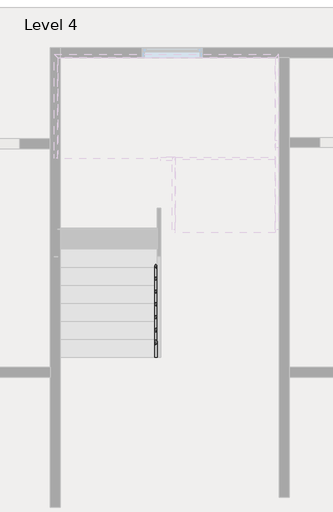
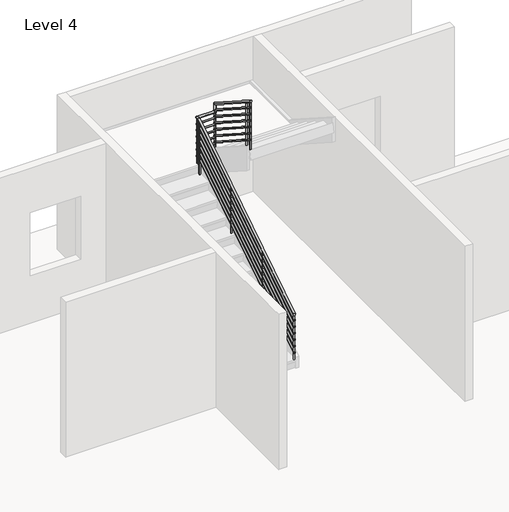
# One storey, part 6 of 7: 1 railing.
"""IFC4 building model written with IfcOpenShell, lengths in millimetres."""

from ifc_helpers import new_model, si_unit, point, frame, frame_2d, origin, place, context, project, spatial, circle_curve, ellipse_curve, trimmed, segment, composite_curve, outline, extrude, element, save
from ifc_brep_helpers import plane_surface, cylinder_surface, advanced_brep

model = new_model("IFC4")

# Units and contexts
model_context = context("Model", 3, world=origin())
ifc_project = project(units=[si_unit("LENGTHUNIT", "METRE", prefix="MILLI")], contexts=[model_context])

# Site, building, storey
site = spatial("IfcSite", under=ifc_project)
building = spatial("IfcBuilding", under=site)
storey = spatial("IfcBuildingStorey", under=building, Name="Level 4", Elevation=9500.0)

# Railing
placement = place(None, origin())
element("IfcRailing", 1, ObjectType="900mm Pipe", at=placement, inside=storey, context=model_context, shape_type="SolidModel", body=[
    advanced_brep(
    [(-504.8393676, 4284.7509075, 10552.7068065), (-544.8393676, 4284.7509075, 10552.7068065), (-504.8393676, 7315.616134, 12497.6470588), (-544.8393676, 7315.616134, 12497.6470588), (-504.8393676, 7337.8781803, 12497.6470588), (-544.8393676, 7377.8781803, 12497.6470588), (-201.3120949, 7337.8781803, 12497.6470588), (-201.3120949, 7377.8781803, 12497.6470588)],
    [
        (0, 1, ellipse_curve(frame((-524.8393676, 4284.7509075, 10552.7068065), z_axis=(0.0, -1.0, 0.0), x_axis=(0.0, 0.0, -1.0)), 23.7637817, 20.0)),
        (1, 0, ellipse_curve(frame((-524.8393676, 4284.7509075, 10552.7068065), z_axis=(0.0, -1.0, 0.0), x_axis=(0.0, 0.0, -1.0)), 23.7637817, 20.0)),
        (0, 2),
        (2, 3, ellipse_curve(frame((-524.8393676, 7315.616134, 12497.6470588), z_axis=(0.0, -0.9595876426002529, -0.28140994326585084), x_axis=(0.0, 0.2814099432658509, -0.959587642600253)), 20.8422859, 20.0)),
        (3, 1),
        (3, 2, ellipse_curve(frame((-524.8393676, 7315.616134, 12497.6470588), z_axis=(0.0, -0.9595876426002529, -0.28140994326585084), x_axis=(0.0, 0.2814099432658509, -0.959587642600253)), 20.8422859, 20.0)),
        (2, 4),
        (4, 5, ellipse_curve(frame((-524.8393676, 7357.8781803, 12497.6470588), z_axis=(-0.7071067811865475, -0.7071067811865475, 0.0), x_axis=(0.7071067811865474, -0.7071067811865476, 0.0)), 28.2842712, 20.0)),
        (5, 3),
        (5, 4, ellipse_curve(frame((-524.8393676, 7357.8781803, 12497.6470588), z_axis=(-0.7071067811865475, -0.7071067811865475, 0.0), x_axis=(0.7071067811865474, -0.7071067811865476, 0.0)), 28.2842712, 20.0)),
        (6, 7, ellipse_curve(frame((-201.3120949, 7357.8781803, 12497.6470588), z_axis=(0.7071067811865476, 0.0, 0.7071067811865476), x_axis=(-0.7071067811865474, 0.0, 0.7071067811865476)), 28.2842712, 20.0)),
        (7, 6, ellipse_curve(frame((-201.3120949, 7357.8781803, 12497.6470588), z_axis=(0.7071067811865476, 0.0, 0.7071067811865476), x_axis=(-0.7071067811865474, 0.0, 0.7071067811865476)), 28.2842712, 20.0)),
        (4, 6),
        (7, 5),
    ],
    [
        plane_surface(frame((-524.8393676, 4284.7509075, 10576.4705882), z_axis=(0.0, -1.0, 0.0), x_axis=(0.0, 0.0, 1.0))),
        cylinder_surface(frame((-524.8393676, 4295.5524077, 10559.6382505), z_axis=(0.0, -0.8416168876622212, -0.5400750081254975), x_axis=(-1.0, 0.0, 0.0)), 20.0),
        cylinder_surface(frame((-524.8393676, 7309.7509075, 12497.6470588), z_axis=(0.0, -1.0, 0.0), x_axis=(-1.0, 0.0, 0.0)), 20.0),
        plane_surface(frame((-221.3120949, 7357.8781803, 12517.6470588), z_axis=(0.7071067811865476, 0.0, 0.7071067811865476), x_axis=(0.7071067811865476, 0.0, -0.7071067811865476))),
        cylinder_surface(frame((-524.8393676, 7357.8781803, 12497.6470588), z_axis=(-1.0, 0.0, 0.0), x_axis=(0.0, 1.0, 0.0)), 20.0),
    ],
    [
        (0, [[1, 2]]),
        (1, [[-1, 3, 4, 5]]),
        (1, [[-2, -5, 6, -3]]),
        (2, [[-4, 7, 8, 9]]),
        (2, [[-6, -9, 10, -7]]),
        (3, [[11, 12]]),
        (4, [[-8, 13, -12, 14]]),
        (4, [[-10, -14, -11, -13]]),
    ],
),
    advanced_brep(
    [(-201.3120949, 7337.8781803, 12497.6470588), (-201.3120949, 7377.8781803, 12497.6470588), (-201.3120949, 7337.8781803, 12643.124843), (-201.3120949, 7377.8781803, 12664.9839572)],
    [
        (0, 1, ellipse_curve(frame((-201.3120949, 7357.8781803, 12497.6470588), z_axis=(-0.7071067811865476, 0.0, -0.7071067811865476), x_axis=(0.7071067811865476, 0.0, -0.7071067811865474)), 28.2842712, 20.0)),
        (1, 0, ellipse_curve(frame((-201.3120949, 7357.8781803, 12497.6470588), z_axis=(-0.7071067811865476, 0.0, -0.7071067811865476), x_axis=(0.7071067811865476, 0.0, -0.7071067811865474)), 28.2842712, 20.0)),
        (2, 3, ellipse_curve(frame((-201.3120949, 7357.8781803, 12654.0544001), z_axis=(0.0, -0.47954405004884676, 0.877517808402057), x_axis=(0.0, -0.8775178084020571, -0.47954405004884676)), 22.7915602, 20.0)),
        (3, 2, ellipse_curve(frame((-201.3120949, 7357.8781803, 12654.0544001), z_axis=(0.0, -0.47954405004884676, 0.877517808402057), x_axis=(0.0, -0.8775178084020571, -0.47954405004884676)), 22.7915602, 20.0)),
        (0, 2),
        (3, 1),
    ],
    [
        plane_surface(frame((-201.3120949, 7357.8781803, 12497.6470588), z_axis=(-0.7071067811865476, 0.0, -0.7071067811865476), x_axis=(0.7071067811865476, 0.0, -0.7071067811865476))),
        plane_surface(frame((-201.3120949, 7357.8781803, 12654.0544001), z_axis=(0.0, -0.47954405004884676, 0.877517808402057), x_axis=(1.0, 0.0, 0.0))),
        cylinder_surface(frame((-201.3120949, 7357.8781803, 12497.6470588), z_axis=(0.0, 0.0, -1.0), x_axis=(0.0, 1.0, 0.0)), 20.0),
    ],
    [
        (0, [[1, 2]]),
        (1, [[3, 4]]),
        (2, [[-1, 5, -4, 6]]),
        (2, [[-2, -6, -3, -5]]),
    ],
),
    advanced_brep(
    [(-221.3120949, 7357.8781803, 12654.0544001), (-181.3120949, 7357.8781803, 12654.0544001), (-221.3120949, 6232.4781803, 13376.2362183), (-181.3120949, 6232.4781803, 13376.2362183)],
    [
        (0, 1, ellipse_curve(frame((-201.3120949, 7357.8781803, 12654.0544001), z_axis=(0.0, 0.47954405004884676, -0.877517808402057), x_axis=(0.0, 0.8775178084020568, 0.47954405004884676)), 22.7915602, 20.0)),
        (1, 0, ellipse_curve(frame((-201.3120949, 7357.8781803, 12654.0544001), z_axis=(0.0, 0.47954405004884676, -0.877517808402057), x_axis=(0.0, 0.8775178084020568, 0.47954405004884676)), 22.7915602, 20.0)),
        (2, 3, ellipse_curve(frame((-201.3120949, 6232.4781803, 13376.2362183), z_axis=(0.0, -1.0, 0.0), x_axis=(0.0, 0.0, -1.0)), 23.7637817, 20.0)),
        (3, 2, ellipse_curve(frame((-201.3120949, 6232.4781803, 13376.2362183), z_axis=(0.0, -1.0, 0.0), x_axis=(0.0, 0.0, -1.0)), 23.7637817, 20.0)),
        (0, 2),
        (3, 1),
    ],
    [
        plane_surface(frame((-201.3120949, 7377.8781803, 12664.9839572), z_axis=(0.0, 0.47954405004884676, -0.877517808402057), x_axis=(1.0, 0.0, 0.0))),
        plane_surface(frame((-201.3120949, 6232.4781803, 13400.0), z_axis=(0.0, -1.0, 0.0), x_axis=(0.0, 0.0, -1.0))),
        cylinder_surface(frame((-201.3120949, 7367.0766801, 12648.1516195), z_axis=(0.0, 0.8416168876622208, -0.5400750081254984), x_axis=(1.0, 0.0, 0.0)), 20.0),
    ],
    [
        (0, [[1, 2]]),
        (1, [[3, 4]]),
        (2, [[-1, 5, -4, 6]]),
        (2, [[-2, -6, -3, -5]]),
    ],
),
    advanced_brep(
    [(-539.8393676, 4284.7509075, 10433.647752), (-509.8393676, 4284.7509075, 10433.647752), (-539.8393676, 7309.7509075, 12374.8242225), (-509.8393676, 7309.7509075, 12374.8242225)],
    [
        (0, 1, ellipse_curve(frame((-524.8393676, 4284.7509075, 10433.647752), z_axis=(0.0, -1.0, 0.0), x_axis=(0.0, 0.0, -1.0)), 17.8228363, 15.0)),
        (1, 0, ellipse_curve(frame((-524.8393676, 4284.7509075, 10433.647752), z_axis=(0.0, -1.0, 0.0), x_axis=(0.0, 0.0, -1.0)), 17.8228363, 15.0)),
        (2, 3, ellipse_curve(frame((-524.8393676, 7309.7509075, 12374.8242225), z_axis=(0.0, 1.0, 0.0), x_axis=(0.0, 0.0, -1.0)), 17.8228363, 15.0)),
        (3, 2, ellipse_curve(frame((-524.8393676, 7309.7509075, 12374.8242225), z_axis=(0.0, 1.0, 0.0), x_axis=(0.0, 0.0, -1.0)), 17.8228363, 15.0)),
        (0, 2),
        (3, 1),
    ],
    [
        plane_surface(frame((-524.8393676, 4284.7509075, 10451.4705882), z_axis=(0.0, -1.0, 0.0), x_axis=(0.0, 0.0, 1.0))),
        plane_surface(frame((-524.8393676, 7309.7509075, 12392.6470588), z_axis=(0.0, 1.0, 0.0), x_axis=(0.0, 0.0, 1.0))),
        cylinder_surface(frame((-524.8393676, 4292.8520327, 10438.8463349), z_axis=(0.0, -0.8416168876622212, -0.5400750081254975), x_axis=(1.0, 0.0, 0.0)), 15.0),
    ],
    [
        (0, [[1, 2]]),
        (1, [[3, 4]]),
        (2, [[-1, 5, -4, 6]]),
        (2, [[-2, -6, -3, -5]]),
    ],
),
    advanced_brep(
    [(-539.8393676, 7309.7509075, 12377.6470588), (-509.8393676, 7309.7509075, 12377.6470588), (-539.8393676, 7342.8781803, 12377.6470588), (-509.8393676, 7342.8781803, 12377.6470588)],
    [
        (0, 1, circle_curve(frame((-524.8393676, 7309.7509075, 12377.6470588), z_axis=(0.0, -1.0, 0.0), x_axis=(1.0, 0.0, 0.0)), 15.0)),
        (1, 0, circle_curve(frame((-524.8393676, 7309.7509075, 12377.6470588), z_axis=(0.0, -1.0, 0.0), x_axis=(1.0, 0.0, 0.0)), 15.0)),
        (2, 3, circle_curve(frame((-524.8393676, 7342.8781803, 12377.6470588), z_axis=(0.0, 1.0, 0.0), x_axis=(1.0, 0.0, 0.0)), 15.0)),
        (3, 2, circle_curve(frame((-524.8393676, 7342.8781803, 12377.6470588), z_axis=(0.0, 1.0, 0.0), x_axis=(1.0, 0.0, 0.0)), 15.0)),
        (0, 2),
        (3, 1),
    ],
    [
        plane_surface(frame((-524.8393676, 7309.7509075, 12392.6470588), z_axis=(0.0, -1.0, 0.0), x_axis=(0.0, 0.0, 1.0))),
        plane_surface(frame((-524.8393676, 7342.8781803, 12392.6470588), z_axis=(0.0, 1.0, 0.0), x_axis=(0.0, 0.0, 1.0))),
        cylinder_surface(frame((-524.8393676, 7309.7509075, 12377.6470588), z_axis=(0.0, -1.0, 0.0), x_axis=(1.0, 0.0, 0.0)), 15.0),
    ],
    [
        (0, [[1, 2]]),
        (1, [[3, 4]]),
        (2, [[-1, 5, -4, 6]]),
        (2, [[-2, -6, -3, -5]]),
    ],
),
    advanced_brep(
    [(-539.8393676, 7372.8781803, 12377.6470588), (-539.8393676, 7342.8781803, 12377.6470588), (-216.3120949, 7372.8781803, 12377.6470588), (-216.3120949, 7342.8781803, 12377.6470588)],
    [
        (0, 1, circle_curve(frame((-539.8393676, 7357.8781803, 12377.6470588), z_axis=(-1.0, 0.0, 0.0), x_axis=(0.0, -1.0, 0.0)), 15.0)),
        (1, 0, circle_curve(frame((-539.8393676, 7357.8781803, 12377.6470588), z_axis=(-1.0, 0.0, 0.0), x_axis=(0.0, -1.0, 0.0)), 15.0)),
        (2, 3, circle_curve(frame((-216.3120949, 7357.8781803, 12377.6470588), z_axis=(1.0, 0.0, 0.0), x_axis=(0.0, -1.0, 0.0)), 15.0)),
        (3, 2, circle_curve(frame((-216.3120949, 7357.8781803, 12377.6470588), z_axis=(1.0, 0.0, 0.0), x_axis=(0.0, -1.0, 0.0)), 15.0)),
        (0, 2),
        (3, 1),
    ],
    [
        plane_surface(frame((-539.8393676, 7357.8781803, 12392.6470588), z_axis=(-1.0, 0.0, 0.0), x_axis=(0.0, 1.0, 0.0))),
        plane_surface(frame((-216.3120949, 7357.8781803, 12392.6470588), z_axis=(1.0, 0.0, 0.0), x_axis=(0.0, 1.0, 0.0))),
        cylinder_surface(frame((-539.8393676, 7357.8781803, 12377.6470588), z_axis=(-1.0, 0.0, 0.0), x_axis=(0.0, -1.0, 0.0)), 15.0),
    ],
    [
        (0, [[1, 2]]),
        (1, [[3, 4]]),
        (2, [[-1, 5, -4, 6]]),
        (2, [[-2, -6, -3, -5]]),
    ],
),
    advanced_brep(
    [(-186.3120949, 7372.8781803, 12525.3696771), (-216.3120949, 7372.8781803, 12525.3696771), (-186.3120949, 6232.4781803, 13257.1771637), (-216.3120949, 6232.4781803, 13257.1771637)],
    [
        (0, 1, ellipse_curve(frame((-201.3120949, 7372.8781803, 12525.3696771), z_axis=(0.0, 1.0, 0.0), x_axis=(0.0, 0.0, -1.0)), 17.8228363, 15.0)),
        (1, 0, ellipse_curve(frame((-201.3120949, 7372.8781803, 12525.3696771), z_axis=(0.0, 1.0, 0.0), x_axis=(0.0, 0.0, -1.0)), 17.8228363, 15.0)),
        (2, 3, ellipse_curve(frame((-201.3120949, 6232.4781803, 13257.1771637), z_axis=(0.0, -1.0, 0.0), x_axis=(0.0, 0.0, -1.0)), 17.8228363, 15.0)),
        (3, 2, ellipse_curve(frame((-201.3120949, 6232.4781803, 13257.1771637), z_axis=(0.0, -1.0, 0.0), x_axis=(0.0, 0.0, -1.0)), 17.8228363, 15.0)),
        (0, 2),
        (3, 1),
    ],
    [
        plane_surface(frame((-201.3120949, 7372.8781803, 12543.1925134), z_axis=(0.0, 1.0, 0.0), x_axis=(0.0, 0.0, -1.0))),
        plane_surface(frame((-201.3120949, 6232.4781803, 13275.0), z_axis=(0.0, -1.0, 0.0), x_axis=(0.0, 0.0, -1.0))),
        cylinder_surface(frame((-201.3120949, 7364.7770552, 12530.5682601), z_axis=(0.0, 0.8416168876622208, -0.5400750081254984), x_axis=(-1.0, 0.0, 0.0)), 15.0),
    ],
    [
        (0, [[1, 2]]),
        (1, [[3, 4]]),
        (2, [[-1, 5, -4, 6]]),
        (2, [[-2, -6, -3, -5]]),
    ],
),
    advanced_brep(
    [(-539.8393676, 4284.7509075, 10308.647752), (-509.8393676, 4284.7509075, 10308.647752), (-539.8393676, 7309.7509075, 12249.8242225), (-509.8393676, 7309.7509075, 12249.8242225)],
    [
        (0, 1, ellipse_curve(frame((-524.8393676, 4284.7509075, 10308.647752), z_axis=(0.0, -1.0, 0.0), x_axis=(0.0, 0.0, -1.0)), 17.8228363, 15.0)),
        (1, 0, ellipse_curve(frame((-524.8393676, 4284.7509075, 10308.647752), z_axis=(0.0, -1.0, 0.0), x_axis=(0.0, 0.0, -1.0)), 17.8228363, 15.0)),
        (2, 3, ellipse_curve(frame((-524.8393676, 7309.7509075, 12249.8242225), z_axis=(0.0, 1.0, 0.0), x_axis=(0.0, 0.0, -1.0)), 17.8228363, 15.0)),
        (3, 2, ellipse_curve(frame((-524.8393676, 7309.7509075, 12249.8242225), z_axis=(0.0, 1.0, 0.0), x_axis=(0.0, 0.0, -1.0)), 17.8228363, 15.0)),
        (0, 2),
        (3, 1),
    ],
    [
        plane_surface(frame((-524.8393676, 4284.7509075, 10326.4705882), z_axis=(0.0, -1.0, 0.0), x_axis=(0.0, 0.0, 1.0))),
        plane_surface(frame((-524.8393676, 7309.7509075, 12267.6470588), z_axis=(0.0, 1.0, 0.0), x_axis=(0.0, 0.0, 1.0))),
        cylinder_surface(frame((-524.8393676, 4292.8520327, 10313.8463349), z_axis=(0.0, -0.8416168876622212, -0.5400750081254975), x_axis=(1.0, 0.0, 0.0)), 15.0),
    ],
    [
        (0, [[1, 2]]),
        (1, [[3, 4]]),
        (2, [[-1, 5, -4, 6]]),
        (2, [[-2, -6, -3, -5]]),
    ],
),
    advanced_brep(
    [(-539.8393676, 7309.7509075, 12252.6470588), (-509.8393676, 7309.7509075, 12252.6470588), (-539.8393676, 7342.8781803, 12252.6470588), (-509.8393676, 7342.8781803, 12252.6470588)],
    [
        (0, 1, circle_curve(frame((-524.8393676, 7309.7509075, 12252.6470588), z_axis=(0.0, -1.0, 0.0), x_axis=(1.0, 0.0, 0.0)), 15.0)),
        (1, 0, circle_curve(frame((-524.8393676, 7309.7509075, 12252.6470588), z_axis=(0.0, -1.0, 0.0), x_axis=(1.0, 0.0, 0.0)), 15.0)),
        (2, 3, circle_curve(frame((-524.8393676, 7342.8781803, 12252.6470588), z_axis=(0.0, 1.0, 0.0), x_axis=(1.0, 0.0, 0.0)), 15.0)),
        (3, 2, circle_curve(frame((-524.8393676, 7342.8781803, 12252.6470588), z_axis=(0.0, 1.0, 0.0), x_axis=(1.0, 0.0, 0.0)), 15.0)),
        (0, 2),
        (3, 1),
    ],
    [
        plane_surface(frame((-524.8393676, 7309.7509075, 12267.6470588), z_axis=(0.0, -1.0, 0.0), x_axis=(0.0, 0.0, 1.0))),
        plane_surface(frame((-524.8393676, 7342.8781803, 12267.6470588), z_axis=(0.0, 1.0, 0.0), x_axis=(0.0, 0.0, 1.0))),
        cylinder_surface(frame((-524.8393676, 7309.7509075, 12252.6470588), z_axis=(0.0, -1.0, 0.0), x_axis=(1.0, 0.0, 0.0)), 15.0),
    ],
    [
        (0, [[1, 2]]),
        (1, [[3, 4]]),
        (2, [[-1, 5, -4, 6]]),
        (2, [[-2, -6, -3, -5]]),
    ],
),
    advanced_brep(
    [(-539.8393676, 7372.8781803, 12252.6470588), (-539.8393676, 7342.8781803, 12252.6470588), (-216.3120949, 7372.8781803, 12252.6470588), (-216.3120949, 7342.8781803, 12252.6470588)],
    [
        (0, 1, circle_curve(frame((-539.8393676, 7357.8781803, 12252.6470588), z_axis=(-1.0, 0.0, 0.0), x_axis=(0.0, -1.0, 0.0)), 15.0)),
        (1, 0, circle_curve(frame((-539.8393676, 7357.8781803, 12252.6470588), z_axis=(-1.0, 0.0, 0.0), x_axis=(0.0, -1.0, 0.0)), 15.0)),
        (2, 3, circle_curve(frame((-216.3120949, 7357.8781803, 12252.6470588), z_axis=(1.0, 0.0, 0.0), x_axis=(0.0, -1.0, 0.0)), 15.0)),
        (3, 2, circle_curve(frame((-216.3120949, 7357.8781803, 12252.6470588), z_axis=(1.0, 0.0, 0.0), x_axis=(0.0, -1.0, 0.0)), 15.0)),
        (0, 2),
        (3, 1),
    ],
    [
        plane_surface(frame((-539.8393676, 7357.8781803, 12267.6470588), z_axis=(-1.0, 0.0, 0.0), x_axis=(0.0, 1.0, 0.0))),
        plane_surface(frame((-216.3120949, 7357.8781803, 12267.6470588), z_axis=(1.0, 0.0, 0.0), x_axis=(0.0, 1.0, 0.0))),
        cylinder_surface(frame((-539.8393676, 7357.8781803, 12252.6470588), z_axis=(-1.0, 0.0, 0.0), x_axis=(0.0, -1.0, 0.0)), 15.0),
    ],
    [
        (0, [[1, 2]]),
        (1, [[3, 4]]),
        (2, [[-1, 5, -4, 6]]),
        (2, [[-2, -6, -3, -5]]),
    ],
),
    advanced_brep(
    [(-186.3120949, 7372.8781803, 12400.3696771), (-216.3120949, 7372.8781803, 12400.3696771), (-186.3120949, 6232.4781803, 13132.1771637), (-216.3120949, 6232.4781803, 13132.1771637)],
    [
        (0, 1, ellipse_curve(frame((-201.3120949, 7372.8781803, 12400.3696771), z_axis=(0.0, 1.0, 0.0), x_axis=(0.0, 0.0, -1.0)), 17.8228363, 15.0)),
        (1, 0, ellipse_curve(frame((-201.3120949, 7372.8781803, 12400.3696771), z_axis=(0.0, 1.0, 0.0), x_axis=(0.0, 0.0, -1.0)), 17.8228363, 15.0)),
        (2, 3, ellipse_curve(frame((-201.3120949, 6232.4781803, 13132.1771637), z_axis=(0.0, -1.0, 0.0), x_axis=(0.0, 0.0, -1.0)), 17.8228363, 15.0)),
        (3, 2, ellipse_curve(frame((-201.3120949, 6232.4781803, 13132.1771637), z_axis=(0.0, -1.0, 0.0), x_axis=(0.0, 0.0, -1.0)), 17.8228363, 15.0)),
        (0, 2),
        (3, 1),
    ],
    [
        plane_surface(frame((-201.3120949, 7372.8781803, 12418.1925134), z_axis=(0.0, 1.0, 0.0), x_axis=(0.0, 0.0, -1.0))),
        plane_surface(frame((-201.3120949, 6232.4781803, 13150.0), z_axis=(0.0, -1.0, 0.0), x_axis=(0.0, 0.0, -1.0))),
        cylinder_surface(frame((-201.3120949, 7364.7770552, 12405.5682601), z_axis=(0.0, 0.8416168876622208, -0.5400750081254984), x_axis=(-1.0, 0.0, 0.0)), 15.0),
    ],
    [
        (0, [[1, 2]]),
        (1, [[3, 4]]),
        (2, [[-1, 5, -4, 6]]),
        (2, [[-2, -6, -3, -5]]),
    ],
),
    advanced_brep(
    [(-539.8393676, 4284.7509075, 10183.647752), (-509.8393676, 4284.7509075, 10183.647752), (-539.8393676, 7309.7509075, 12124.8242225), (-509.8393676, 7309.7509075, 12124.8242225)],
    [
        (0, 1, ellipse_curve(frame((-524.8393676, 4284.7509075, 10183.647752), z_axis=(0.0, -1.0, 0.0), x_axis=(0.0, 0.0, -1.0)), 17.8228363, 15.0)),
        (1, 0, ellipse_curve(frame((-524.8393676, 4284.7509075, 10183.647752), z_axis=(0.0, -1.0, 0.0), x_axis=(0.0, 0.0, -1.0)), 17.8228363, 15.0)),
        (2, 3, ellipse_curve(frame((-524.8393676, 7309.7509075, 12124.8242225), z_axis=(0.0, 1.0, 0.0), x_axis=(0.0, 0.0, -1.0)), 17.8228363, 15.0)),
        (3, 2, ellipse_curve(frame((-524.8393676, 7309.7509075, 12124.8242225), z_axis=(0.0, 1.0, 0.0), x_axis=(0.0, 0.0, -1.0)), 17.8228363, 15.0)),
        (0, 2),
        (3, 1),
    ],
    [
        plane_surface(frame((-524.8393676, 4284.7509075, 10201.4705882), z_axis=(0.0, -1.0, 0.0), x_axis=(0.0, 0.0, 1.0))),
        plane_surface(frame((-524.8393676, 7309.7509075, 12142.6470588), z_axis=(0.0, 1.0, 0.0), x_axis=(0.0, 0.0, 1.0))),
        cylinder_surface(frame((-524.8393676, 4292.8520327, 10188.8463349), z_axis=(0.0, -0.8416168876622212, -0.5400750081254975), x_axis=(1.0, 0.0, 0.0)), 15.0),
    ],
    [
        (0, [[1, 2]]),
        (1, [[3, 4]]),
        (2, [[-1, 5, -4, 6]]),
        (2, [[-2, -6, -3, -5]]),
    ],
),
    advanced_brep(
    [(-539.8393676, 7309.7509075, 12127.6470588), (-509.8393676, 7309.7509075, 12127.6470588), (-539.8393676, 7342.8781803, 12127.6470588), (-509.8393676, 7342.8781803, 12127.6470588)],
    [
        (0, 1, circle_curve(frame((-524.8393676, 7309.7509075, 12127.6470588), z_axis=(0.0, -1.0, 0.0), x_axis=(1.0, 0.0, 0.0)), 15.0)),
        (1, 0, circle_curve(frame((-524.8393676, 7309.7509075, 12127.6470588), z_axis=(0.0, -1.0, 0.0), x_axis=(1.0, 0.0, 0.0)), 15.0)),
        (2, 3, circle_curve(frame((-524.8393676, 7342.8781803, 12127.6470588), z_axis=(0.0, 1.0, 0.0), x_axis=(1.0, 0.0, 0.0)), 15.0)),
        (3, 2, circle_curve(frame((-524.8393676, 7342.8781803, 12127.6470588), z_axis=(0.0, 1.0, 0.0), x_axis=(1.0, 0.0, 0.0)), 15.0)),
        (0, 2),
        (3, 1),
    ],
    [
        plane_surface(frame((-524.8393676, 7309.7509075, 12142.6470588), z_axis=(0.0, -1.0, 0.0), x_axis=(0.0, 0.0, 1.0))),
        plane_surface(frame((-524.8393676, 7342.8781803, 12142.6470588), z_axis=(0.0, 1.0, 0.0), x_axis=(0.0, 0.0, 1.0))),
        cylinder_surface(frame((-524.8393676, 7309.7509075, 12127.6470588), z_axis=(0.0, -1.0, 0.0), x_axis=(1.0, 0.0, 0.0)), 15.0),
    ],
    [
        (0, [[1, 2]]),
        (1, [[3, 4]]),
        (2, [[-1, 5, -4, 6]]),
        (2, [[-2, -6, -3, -5]]),
    ],
),
    advanced_brep(
    [(-539.8393676, 7372.8781803, 12127.6470588), (-539.8393676, 7342.8781803, 12127.6470588), (-216.3120949, 7372.8781803, 12127.6470588), (-216.3120949, 7342.8781803, 12127.6470588)],
    [
        (0, 1, circle_curve(frame((-539.8393676, 7357.8781803, 12127.6470588), z_axis=(-1.0, 0.0, 0.0), x_axis=(0.0, -1.0, 0.0)), 15.0)),
        (1, 0, circle_curve(frame((-539.8393676, 7357.8781803, 12127.6470588), z_axis=(-1.0, 0.0, 0.0), x_axis=(0.0, -1.0, 0.0)), 15.0)),
        (2, 3, circle_curve(frame((-216.3120949, 7357.8781803, 12127.6470588), z_axis=(1.0, 0.0, 0.0), x_axis=(0.0, -1.0, 0.0)), 15.0)),
        (3, 2, circle_curve(frame((-216.3120949, 7357.8781803, 12127.6470588), z_axis=(1.0, 0.0, 0.0), x_axis=(0.0, -1.0, 0.0)), 15.0)),
        (0, 2),
        (3, 1),
    ],
    [
        plane_surface(frame((-539.8393676, 7357.8781803, 12142.6470588), z_axis=(-1.0, 0.0, 0.0), x_axis=(0.0, 1.0, 0.0))),
        plane_surface(frame((-216.3120949, 7357.8781803, 12142.6470588), z_axis=(1.0, 0.0, 0.0), x_axis=(0.0, 1.0, 0.0))),
        cylinder_surface(frame((-539.8393676, 7357.8781803, 12127.6470588), z_axis=(-1.0, 0.0, 0.0), x_axis=(0.0, -1.0, 0.0)), 15.0),
    ],
    [
        (0, [[1, 2]]),
        (1, [[3, 4]]),
        (2, [[-1, 5, -4, 6]]),
        (2, [[-2, -6, -3, -5]]),
    ],
),
    advanced_brep(
    [(-186.3120949, 7372.8781803, 12275.3696771), (-216.3120949, 7372.8781803, 12275.3696771), (-186.3120949, 6232.4781803, 13007.1771637), (-216.3120949, 6232.4781803, 13007.1771637)],
    [
        (0, 1, ellipse_curve(frame((-201.3120949, 7372.8781803, 12275.3696771), z_axis=(0.0, 1.0, 0.0), x_axis=(0.0, 0.0, -1.0)), 17.8228363, 15.0)),
        (1, 0, ellipse_curve(frame((-201.3120949, 7372.8781803, 12275.3696771), z_axis=(0.0, 1.0, 0.0), x_axis=(0.0, 0.0, -1.0)), 17.8228363, 15.0)),
        (2, 3, ellipse_curve(frame((-201.3120949, 6232.4781803, 13007.1771637), z_axis=(0.0, -1.0, 0.0), x_axis=(0.0, 0.0, -1.0)), 17.8228363, 15.0)),
        (3, 2, ellipse_curve(frame((-201.3120949, 6232.4781803, 13007.1771637), z_axis=(0.0, -1.0, 0.0), x_axis=(0.0, 0.0, -1.0)), 17.8228363, 15.0)),
        (0, 2),
        (3, 1),
    ],
    [
        plane_surface(frame((-201.3120949, 7372.8781803, 12293.1925134), z_axis=(0.0, 1.0, 0.0), x_axis=(0.0, 0.0, -1.0))),
        plane_surface(frame((-201.3120949, 6232.4781803, 13025.0), z_axis=(0.0, -1.0, 0.0), x_axis=(0.0, 0.0, -1.0))),
        cylinder_surface(frame((-201.3120949, 7364.7770552, 12280.5682601), z_axis=(0.0, 0.8416168876622208, -0.5400750081254984), x_axis=(-1.0, 0.0, 0.0)), 15.0),
    ],
    [
        (0, [[1, 2]]),
        (1, [[3, 4]]),
        (2, [[-1, 5, -4, 6]]),
        (2, [[-2, -6, -3, -5]]),
    ],
),
    advanced_brep(
    [(-539.8393676, 4284.7509075, 10058.647752), (-509.8393676, 4284.7509075, 10058.647752), (-539.8393676, 7309.7509075, 11999.8242225), (-509.8393676, 7309.7509075, 11999.8242225)],
    [
        (0, 1, ellipse_curve(frame((-524.8393676, 4284.7509075, 10058.647752), z_axis=(0.0, -1.0, 0.0), x_axis=(0.0, 0.0, -1.0)), 17.8228363, 15.0)),
        (1, 0, ellipse_curve(frame((-524.8393676, 4284.7509075, 10058.647752), z_axis=(0.0, -1.0, 0.0), x_axis=(0.0, 0.0, -1.0)), 17.8228363, 15.0)),
        (2, 3, ellipse_curve(frame((-524.8393676, 7309.7509075, 11999.8242225), z_axis=(0.0, 1.0, 0.0), x_axis=(0.0, 0.0, -1.0)), 17.8228363, 15.0)),
        (3, 2, ellipse_curve(frame((-524.8393676, 7309.7509075, 11999.8242225), z_axis=(0.0, 1.0, 0.0), x_axis=(0.0, 0.0, -1.0)), 17.8228363, 15.0)),
        (0, 2),
        (3, 1),
    ],
    [
        plane_surface(frame((-524.8393676, 4284.7509075, 10076.4705882), z_axis=(0.0, -1.0, 0.0), x_axis=(0.0, 0.0, 1.0))),
        plane_surface(frame((-524.8393676, 7309.7509075, 12017.6470588), z_axis=(0.0, 1.0, 0.0), x_axis=(0.0, 0.0, 1.0))),
        cylinder_surface(frame((-524.8393676, 4292.8520327, 10063.8463349), z_axis=(0.0, -0.8416168876622212, -0.5400750081254975), x_axis=(1.0, 0.0, 0.0)), 15.0),
    ],
    [
        (0, [[1, 2]]),
        (1, [[3, 4]]),
        (2, [[-1, 5, -4, 6]]),
        (2, [[-2, -6, -3, -5]]),
    ],
),
    advanced_brep(
    [(-539.8393676, 7309.7509075, 12002.6470588), (-509.8393676, 7309.7509075, 12002.6470588), (-539.8393676, 7342.8781803, 12002.6470588), (-509.8393676, 7342.8781803, 12002.6470588)],
    [
        (0, 1, circle_curve(frame((-524.8393676, 7309.7509075, 12002.6470588), z_axis=(0.0, -1.0, 0.0), x_axis=(1.0, 0.0, 0.0)), 15.0)),
        (1, 0, circle_curve(frame((-524.8393676, 7309.7509075, 12002.6470588), z_axis=(0.0, -1.0, 0.0), x_axis=(1.0, 0.0, 0.0)), 15.0)),
        (2, 3, circle_curve(frame((-524.8393676, 7342.8781803, 12002.6470588), z_axis=(0.0, 1.0, 0.0), x_axis=(1.0, 0.0, 0.0)), 15.0)),
        (3, 2, circle_curve(frame((-524.8393676, 7342.8781803, 12002.6470588), z_axis=(0.0, 1.0, 0.0), x_axis=(1.0, 0.0, 0.0)), 15.0)),
        (0, 2),
        (3, 1),
    ],
    [
        plane_surface(frame((-524.8393676, 7309.7509075, 12017.6470588), z_axis=(0.0, -1.0, 0.0), x_axis=(0.0, 0.0, 1.0))),
        plane_surface(frame((-524.8393676, 7342.8781803, 12017.6470588), z_axis=(0.0, 1.0, 0.0), x_axis=(0.0, 0.0, 1.0))),
        cylinder_surface(frame((-524.8393676, 7309.7509075, 12002.6470588), z_axis=(0.0, -1.0, 0.0), x_axis=(1.0, 0.0, 0.0)), 15.0),
    ],
    [
        (0, [[1, 2]]),
        (1, [[3, 4]]),
        (2, [[-1, 5, -4, 6]]),
        (2, [[-2, -6, -3, -5]]),
    ],
),
    advanced_brep(
    [(-539.8393676, 7372.8781803, 12002.6470588), (-539.8393676, 7342.8781803, 12002.6470588), (-216.3120949, 7372.8781803, 12002.6470588), (-216.3120949, 7342.8781803, 12002.6470588)],
    [
        (0, 1, circle_curve(frame((-539.8393676, 7357.8781803, 12002.6470588), z_axis=(-1.0, 0.0, 0.0), x_axis=(0.0, -1.0, 0.0)), 15.0)),
        (1, 0, circle_curve(frame((-539.8393676, 7357.8781803, 12002.6470588), z_axis=(-1.0, 0.0, 0.0), x_axis=(0.0, -1.0, 0.0)), 15.0)),
        (2, 3, circle_curve(frame((-216.3120949, 7357.8781803, 12002.6470588), z_axis=(1.0, 0.0, 0.0), x_axis=(0.0, -1.0, 0.0)), 15.0)),
        (3, 2, circle_curve(frame((-216.3120949, 7357.8781803, 12002.6470588), z_axis=(1.0, 0.0, 0.0), x_axis=(0.0, -1.0, 0.0)), 15.0)),
        (0, 2),
        (3, 1),
    ],
    [
        plane_surface(frame((-539.8393676, 7357.8781803, 12017.6470588), z_axis=(-1.0, 0.0, 0.0), x_axis=(0.0, 1.0, 0.0))),
        plane_surface(frame((-216.3120949, 7357.8781803, 12017.6470588), z_axis=(1.0, 0.0, 0.0), x_axis=(0.0, 1.0, 0.0))),
        cylinder_surface(frame((-539.8393676, 7357.8781803, 12002.6470588), z_axis=(-1.0, 0.0, 0.0), x_axis=(0.0, -1.0, 0.0)), 15.0),
    ],
    [
        (0, [[1, 2]]),
        (1, [[3, 4]]),
        (2, [[-1, 5, -4, 6]]),
        (2, [[-2, -6, -3, -5]]),
    ],
),
    advanced_brep(
    [(-186.3120949, 7372.8781803, 12150.3696771), (-216.3120949, 7372.8781803, 12150.3696771), (-186.3120949, 6232.4781803, 12882.1771637), (-216.3120949, 6232.4781803, 12882.1771637)],
    [
        (0, 1, ellipse_curve(frame((-201.3120949, 7372.8781803, 12150.3696771), z_axis=(0.0, 1.0, 0.0), x_axis=(0.0, 0.0, -1.0)), 17.8228363, 15.0)),
        (1, 0, ellipse_curve(frame((-201.3120949, 7372.8781803, 12150.3696771), z_axis=(0.0, 1.0, 0.0), x_axis=(0.0, 0.0, -1.0)), 17.8228363, 15.0)),
        (2, 3, ellipse_curve(frame((-201.3120949, 6232.4781803, 12882.1771637), z_axis=(0.0, -1.0, 0.0), x_axis=(0.0, 0.0, -1.0)), 17.8228363, 15.0)),
        (3, 2, ellipse_curve(frame((-201.3120949, 6232.4781803, 12882.1771637), z_axis=(0.0, -1.0, 0.0), x_axis=(0.0, 0.0, -1.0)), 17.8228363, 15.0)),
        (0, 2),
        (3, 1),
    ],
    [
        plane_surface(frame((-201.3120949, 7372.8781803, 12168.1925134), z_axis=(0.0, 1.0, 0.0), x_axis=(0.0, 0.0, -1.0))),
        plane_surface(frame((-201.3120949, 6232.4781803, 12900.0), z_axis=(0.0, -1.0, 0.0), x_axis=(0.0, 0.0, -1.0))),
        cylinder_surface(frame((-201.3120949, 7364.7770552, 12155.5682601), z_axis=(0.0, 0.8416168876622208, -0.5400750081254984), x_axis=(-1.0, 0.0, 0.0)), 15.0),
    ],
    [
        (0, [[1, 2]]),
        (1, [[3, 4]]),
        (2, [[-1, 5, -4, 6]]),
        (2, [[-2, -6, -3, -5]]),
    ],
),
    advanced_brep(
    [(-539.8393676, 4284.7509075, 9933.647752), (-509.8393676, 4284.7509075, 9933.647752), (-539.8393676, 7309.7509075, 11874.8242225), (-509.8393676, 7309.7509075, 11874.8242225)],
    [
        (0, 1, ellipse_curve(frame((-524.8393676, 4284.7509075, 9933.647752), z_axis=(0.0, -1.0, 0.0), x_axis=(0.0, 0.0, -1.0)), 17.8228363, 15.0)),
        (1, 0, ellipse_curve(frame((-524.8393676, 4284.7509075, 9933.647752), z_axis=(0.0, -1.0, 0.0), x_axis=(0.0, 0.0, -1.0)), 17.8228363, 15.0)),
        (2, 3, ellipse_curve(frame((-524.8393676, 7309.7509075, 11874.8242225), z_axis=(0.0, 1.0, 0.0), x_axis=(0.0, 0.0, -1.0)), 17.8228363, 15.0)),
        (3, 2, ellipse_curve(frame((-524.8393676, 7309.7509075, 11874.8242225), z_axis=(0.0, 1.0, 0.0), x_axis=(0.0, 0.0, -1.0)), 17.8228363, 15.0)),
        (0, 2),
        (3, 1),
    ],
    [
        plane_surface(frame((-524.8393676, 4284.7509075, 9951.4705882), z_axis=(0.0, -1.0, 0.0), x_axis=(0.0, 0.0, 1.0))),
        plane_surface(frame((-524.8393676, 7309.7509075, 11892.6470588), z_axis=(0.0, 1.0, 0.0), x_axis=(0.0, 0.0, 1.0))),
        cylinder_surface(frame((-524.8393676, 4292.8520327, 9938.8463349), z_axis=(0.0, -0.8416168876622212, -0.5400750081254975), x_axis=(1.0, 0.0, 0.0)), 15.0),
    ],
    [
        (0, [[1, 2]]),
        (1, [[3, 4]]),
        (2, [[-1, 5, -4, 6]]),
        (2, [[-2, -6, -3, -5]]),
    ],
),
    advanced_brep(
    [(-539.8393676, 7309.7509075, 11877.6470588), (-509.8393676, 7309.7509075, 11877.6470588), (-539.8393676, 7342.8781803, 11877.6470588), (-509.8393676, 7342.8781803, 11877.6470588)],
    [
        (0, 1, circle_curve(frame((-524.8393676, 7309.7509075, 11877.6470588), z_axis=(0.0, -1.0, 0.0), x_axis=(1.0, 0.0, 0.0)), 15.0)),
        (1, 0, circle_curve(frame((-524.8393676, 7309.7509075, 11877.6470588), z_axis=(0.0, -1.0, 0.0), x_axis=(1.0, 0.0, 0.0)), 15.0)),
        (2, 3, circle_curve(frame((-524.8393676, 7342.8781803, 11877.6470588), z_axis=(0.0, 1.0, 0.0), x_axis=(1.0, 0.0, 0.0)), 15.0)),
        (3, 2, circle_curve(frame((-524.8393676, 7342.8781803, 11877.6470588), z_axis=(0.0, 1.0, 0.0), x_axis=(1.0, 0.0, 0.0)), 15.0)),
        (0, 2),
        (3, 1),
    ],
    [
        plane_surface(frame((-524.8393676, 7309.7509075, 11892.6470588), z_axis=(0.0, -1.0, 0.0), x_axis=(0.0, 0.0, 1.0))),
        plane_surface(frame((-524.8393676, 7342.8781803, 11892.6470588), z_axis=(0.0, 1.0, 0.0), x_axis=(0.0, 0.0, 1.0))),
        cylinder_surface(frame((-524.8393676, 7309.7509075, 11877.6470588), z_axis=(0.0, -1.0, 0.0), x_axis=(1.0, 0.0, 0.0)), 15.0),
    ],
    [
        (0, [[1, 2]]),
        (1, [[3, 4]]),
        (2, [[-1, 5, -4, 6]]),
        (2, [[-2, -6, -3, -5]]),
    ],
),
    advanced_brep(
    [(-539.8393676, 7372.8781803, 11877.6470588), (-539.8393676, 7342.8781803, 11877.6470588), (-216.3120949, 7372.8781803, 11877.6470588), (-216.3120949, 7342.8781803, 11877.6470588)],
    [
        (0, 1, circle_curve(frame((-539.8393676, 7357.8781803, 11877.6470588), z_axis=(-1.0, 0.0, 0.0), x_axis=(0.0, -1.0, 0.0)), 15.0)),
        (1, 0, circle_curve(frame((-539.8393676, 7357.8781803, 11877.6470588), z_axis=(-1.0, 0.0, 0.0), x_axis=(0.0, -1.0, 0.0)), 15.0)),
        (2, 3, circle_curve(frame((-216.3120949, 7357.8781803, 11877.6470588), z_axis=(1.0, 0.0, 0.0), x_axis=(0.0, -1.0, 0.0)), 15.0)),
        (3, 2, circle_curve(frame((-216.3120949, 7357.8781803, 11877.6470588), z_axis=(1.0, 0.0, 0.0), x_axis=(0.0, -1.0, 0.0)), 15.0)),
        (0, 2),
        (3, 1),
    ],
    [
        plane_surface(frame((-539.8393676, 7357.8781803, 11892.6470588), z_axis=(-1.0, 0.0, 0.0), x_axis=(0.0, 1.0, 0.0))),
        plane_surface(frame((-216.3120949, 7357.8781803, 11892.6470588), z_axis=(1.0, 0.0, 0.0), x_axis=(0.0, 1.0, 0.0))),
        cylinder_surface(frame((-539.8393676, 7357.8781803, 11877.6470588), z_axis=(-1.0, 0.0, 0.0), x_axis=(0.0, -1.0, 0.0)), 15.0),
    ],
    [
        (0, [[1, 2]]),
        (1, [[3, 4]]),
        (2, [[-1, 5, -4, 6]]),
        (2, [[-2, -6, -3, -5]]),
    ],
),
    advanced_brep(
    [(-186.3120949, 7372.8781803, 12025.3696771), (-216.3120949, 7372.8781803, 12025.3696771), (-186.3120949, 6232.4781803, 12757.1771637), (-216.3120949, 6232.4781803, 12757.1771637)],
    [
        (0, 1, ellipse_curve(frame((-201.3120949, 7372.8781803, 12025.3696771), z_axis=(0.0, 1.0, 0.0), x_axis=(0.0, 0.0, -1.0)), 17.8228363, 15.0)),
        (1, 0, ellipse_curve(frame((-201.3120949, 7372.8781803, 12025.3696771), z_axis=(0.0, 1.0, 0.0), x_axis=(0.0, 0.0, -1.0)), 17.8228363, 15.0)),
        (2, 3, ellipse_curve(frame((-201.3120949, 6232.4781803, 12757.1771637), z_axis=(0.0, -1.0, 0.0), x_axis=(0.0, 0.0, -1.0)), 17.8228363, 15.0)),
        (3, 2, ellipse_curve(frame((-201.3120949, 6232.4781803, 12757.1771637), z_axis=(0.0, -1.0, 0.0), x_axis=(0.0, 0.0, -1.0)), 17.8228363, 15.0)),
        (0, 2),
        (3, 1),
    ],
    [
        plane_surface(frame((-201.3120949, 7372.8781803, 12043.1925134), z_axis=(0.0, 1.0, 0.0), x_axis=(0.0, 0.0, -1.0))),
        plane_surface(frame((-201.3120949, 6232.4781803, 12775.0), z_axis=(0.0, -1.0, 0.0), x_axis=(0.0, 0.0, -1.0))),
        cylinder_surface(frame((-201.3120949, 7364.7770552, 12030.5682601), z_axis=(0.0, 0.8416168876622208, -0.5400750081254984), x_axis=(-1.0, 0.0, 0.0)), 15.0),
    ],
    [
        (0, [[1, 2]]),
        (1, [[3, 4]]),
        (2, [[-1, 5, -4, 6]]),
        (2, [[-2, -6, -3, -5]]),
    ],
),
    advanced_brep(
    [(-539.8393676, 4284.7509075, 9808.647752), (-509.8393676, 4284.7509075, 9808.647752), (-539.8393676, 7309.7509075, 11749.8242225), (-509.8393676, 7309.7509075, 11749.8242225)],
    [
        (0, 1, ellipse_curve(frame((-524.8393676, 4284.7509075, 9808.647752), z_axis=(0.0, -1.0, 0.0), x_axis=(0.0, 0.0, -1.0)), 17.8228363, 15.0)),
        (1, 0, ellipse_curve(frame((-524.8393676, 4284.7509075, 9808.647752), z_axis=(0.0, -1.0, 0.0), x_axis=(0.0, 0.0, -1.0)), 17.8228363, 15.0)),
        (2, 3, ellipse_curve(frame((-524.8393676, 7309.7509075, 11749.8242225), z_axis=(0.0, 1.0, 0.0), x_axis=(0.0, 0.0, -1.0)), 17.8228363, 15.0)),
        (3, 2, ellipse_curve(frame((-524.8393676, 7309.7509075, 11749.8242225), z_axis=(0.0, 1.0, 0.0), x_axis=(0.0, 0.0, -1.0)), 17.8228363, 15.0)),
        (0, 2),
        (3, 1),
    ],
    [
        plane_surface(frame((-524.8393676, 4284.7509075, 9826.4705882), z_axis=(0.0, -1.0, 0.0), x_axis=(0.0, 0.0, 1.0))),
        plane_surface(frame((-524.8393676, 7309.7509075, 11767.6470588), z_axis=(0.0, 1.0, 0.0), x_axis=(0.0, 0.0, 1.0))),
        cylinder_surface(frame((-524.8393676, 4292.8520327, 9813.8463349), z_axis=(0.0, -0.8416168876622212, -0.5400750081254975), x_axis=(1.0, 0.0, 0.0)), 15.0),
    ],
    [
        (0, [[1, 2]]),
        (1, [[3, 4]]),
        (2, [[-1, 5, -4, 6]]),
        (2, [[-2, -6, -3, -5]]),
    ],
),
    advanced_brep(
    [(-539.8393676, 7309.7509075, 11752.6470588), (-509.8393676, 7309.7509075, 11752.6470588), (-539.8393676, 7342.8781803, 11752.6470588), (-509.8393676, 7342.8781803, 11752.6470588)],
    [
        (0, 1, circle_curve(frame((-524.8393676, 7309.7509075, 11752.6470588), z_axis=(0.0, -1.0, 0.0), x_axis=(1.0, 0.0, 0.0)), 15.0)),
        (1, 0, circle_curve(frame((-524.8393676, 7309.7509075, 11752.6470588), z_axis=(0.0, -1.0, 0.0), x_axis=(1.0, 0.0, 0.0)), 15.0)),
        (2, 3, circle_curve(frame((-524.8393676, 7342.8781803, 11752.6470588), z_axis=(0.0, 1.0, 0.0), x_axis=(1.0, 0.0, 0.0)), 15.0)),
        (3, 2, circle_curve(frame((-524.8393676, 7342.8781803, 11752.6470588), z_axis=(0.0, 1.0, 0.0), x_axis=(1.0, 0.0, 0.0)), 15.0)),
        (0, 2),
        (3, 1),
    ],
    [
        plane_surface(frame((-524.8393676, 7309.7509075, 11767.6470588), z_axis=(0.0, -1.0, 0.0), x_axis=(0.0, 0.0, 1.0))),
        plane_surface(frame((-524.8393676, 7342.8781803, 11767.6470588), z_axis=(0.0, 1.0, 0.0), x_axis=(0.0, 0.0, 1.0))),
        cylinder_surface(frame((-524.8393676, 7309.7509075, 11752.6470588), z_axis=(0.0, -1.0, 0.0), x_axis=(1.0, 0.0, 0.0)), 15.0),
    ],
    [
        (0, [[1, 2]]),
        (1, [[3, 4]]),
        (2, [[-1, 5, -4, 6]]),
        (2, [[-2, -6, -3, -5]]),
    ],
),
    advanced_brep(
    [(-539.8393676, 7372.8781803, 11752.6470588), (-539.8393676, 7342.8781803, 11752.6470588), (-216.3120949, 7372.8781803, 11752.6470588), (-216.3120949, 7342.8781803, 11752.6470588)],
    [
        (0, 1, circle_curve(frame((-539.8393676, 7357.8781803, 11752.6470588), z_axis=(-1.0, 0.0, 0.0), x_axis=(0.0, -1.0, 0.0)), 15.0)),
        (1, 0, circle_curve(frame((-539.8393676, 7357.8781803, 11752.6470588), z_axis=(-1.0, 0.0, 0.0), x_axis=(0.0, -1.0, 0.0)), 15.0)),
        (2, 3, circle_curve(frame((-216.3120949, 7357.8781803, 11752.6470588), z_axis=(1.0, 0.0, 0.0), x_axis=(0.0, -1.0, 0.0)), 15.0)),
        (3, 2, circle_curve(frame((-216.3120949, 7357.8781803, 11752.6470588), z_axis=(1.0, 0.0, 0.0), x_axis=(0.0, -1.0, 0.0)), 15.0)),
        (0, 2),
        (3, 1),
    ],
    [
        plane_surface(frame((-539.8393676, 7357.8781803, 11767.6470588), z_axis=(-1.0, 0.0, 0.0), x_axis=(0.0, 1.0, 0.0))),
        plane_surface(frame((-216.3120949, 7357.8781803, 11767.6470588), z_axis=(1.0, 0.0, 0.0), x_axis=(0.0, 1.0, 0.0))),
        cylinder_surface(frame((-539.8393676, 7357.8781803, 11752.6470588), z_axis=(-1.0, 0.0, 0.0), x_axis=(0.0, -1.0, 0.0)), 15.0),
    ],
    [
        (0, [[1, 2]]),
        (1, [[3, 4]]),
        (2, [[-1, 5, -4, 6]]),
        (2, [[-2, -6, -3, -5]]),
    ],
),
    advanced_brep(
    [(-186.3120949, 7372.8781803, 11900.3696771), (-216.3120949, 7372.8781803, 11900.3696771), (-186.3120949, 6232.4781803, 12632.1771637), (-216.3120949, 6232.4781803, 12632.1771637)],
    [
        (0, 1, ellipse_curve(frame((-201.3120949, 7372.8781803, 11900.3696771), z_axis=(0.0, 1.0, 0.0), x_axis=(0.0, 0.0, -1.0)), 17.8228363, 15.0)),
        (1, 0, ellipse_curve(frame((-201.3120949, 7372.8781803, 11900.3696771), z_axis=(0.0, 1.0, 0.0), x_axis=(0.0, 0.0, -1.0)), 17.8228363, 15.0)),
        (2, 3, ellipse_curve(frame((-201.3120949, 6232.4781803, 12632.1771637), z_axis=(0.0, -1.0, 0.0), x_axis=(0.0, 0.0, -1.0)), 17.8228363, 15.0)),
        (3, 2, ellipse_curve(frame((-201.3120949, 6232.4781803, 12632.1771637), z_axis=(0.0, -1.0, 0.0), x_axis=(0.0, 0.0, -1.0)), 17.8228363, 15.0)),
        (0, 2),
        (3, 1),
    ],
    [
        plane_surface(frame((-201.3120949, 7372.8781803, 11918.1925134), z_axis=(0.0, 1.0, 0.0), x_axis=(0.0, 0.0, -1.0))),
        plane_surface(frame((-201.3120949, 6232.4781803, 12650.0), z_axis=(0.0, -1.0, 0.0), x_axis=(0.0, 0.0, -1.0))),
        cylinder_surface(frame((-201.3120949, 7364.7770552, 11905.5682601), z_axis=(0.0, 0.8416168876622208, -0.5400750081254984), x_axis=(-1.0, 0.0, 0.0)), 15.0),
    ],
    [
        (0, [[1, 2]]),
        (1, [[3, 4]]),
        (2, [[-1, 5, -4, 6]]),
        (2, [[-2, -6, -3, -5]]),
    ],
),
    advanced_brep(
    [(-213.8120949, 6357.8781803, 13272.0018483), (-213.8120949, 6357.8781803, 12323.5294118), (-188.8120949, 6357.8781803, 12323.5294118), (-188.8120949, 6357.8781803, 13272.0018483)],
    [
        (0, 1),
        (1, 2, circle_curve(frame((-201.3120949, 6357.8781803, 12323.5294118), z_axis=(0.0, 0.0, 1.0), x_axis=(1.0, 0.0, 0.0)), 12.5)),
        (2, 3),
        (3, 0, ellipse_curve(frame((-201.3120949, 6357.8781803, 13272.0018483), z_axis=(0.0, -0.5400750081254972, -0.8416168876622213), x_axis=(0.0, -0.8416168876622212, 0.5400750081254974)), 14.8523636, 12.5)),
        (0, 3, ellipse_curve(frame((-201.3120949, 6357.8781803, 13272.0018483), z_axis=(0.0, -0.5400750081254972, -0.8416168876622213), x_axis=(0.0, -0.8416168876622212, 0.5400750081254974)), 14.8523636, 12.5)),
        (2, 1, circle_curve(frame((-201.3120949, 6357.8781803, 12323.5294118), z_axis=(0.0, 0.0, 1.0), x_axis=(1.0, 0.0, 0.0)), 12.5)),
    ],
    [
        cylinder_surface(frame((-201.3120949, 6357.8781803, 12223.5294118), z_axis=(0.0, 0.0, 1.0), x_axis=(1.0, 0.0, 0.0)), 12.5),
        plane_surface(frame((-176.3120949, 6332.8781803, 13288.0446291), z_axis=(0.0, 0.5400750081254972, 0.8416168876622213), x_axis=(-1.0, 0.0, 0.0))),
        plane_surface(frame((-176.3120949, 6382.8781803, 12323.5294118), z_axis=(0.0, 0.0, -1.0), x_axis=(-1.0, 0.0, 0.0))),
    ],
    [
        (0, [[1, 2, 3, 4]]),
        (0, [[-1, 5, -3, 6]]),
        (1, [[-4, -5]]),
        (2, [[-2, -6]]),
    ],
),
    advanced_brep(
    [(-512.3393676, 7284.7509075, 12454.0767147), (-512.3393676, 7284.7509075, 11441.1764706), (-537.3393676, 7284.7509075, 11441.1764706), (-537.3393676, 7284.7509075, 12454.0767147)],
    [
        (0, 1),
        (1, 2, circle_curve(frame((-524.8393676, 7284.7509075, 11441.1764706), z_axis=(0.0, 0.0, 1.0), x_axis=(-1.0, 0.0, 0.0)), 12.5)),
        (2, 3),
        (3, 0, ellipse_curve(frame((-524.8393676, 7284.7509075, 12454.0767147), z_axis=(0.0, 0.5400750081254972, -0.8416168876622213), x_axis=(0.0, 0.8416168876622212, 0.5400750081254974)), 14.8523636, 12.5)),
        (0, 3, ellipse_curve(frame((-524.8393676, 7284.7509075, 12454.0767147), z_axis=(0.0, 0.5400750081254972, -0.8416168876622213), x_axis=(0.0, 0.8416168876622212, 0.5400750081254974)), 14.8523636, 12.5)),
        (2, 1, circle_curve(frame((-524.8393676, 7284.7509075, 11441.1764706), z_axis=(0.0, 0.0, 1.0), x_axis=(-1.0, 0.0, 0.0)), 12.5)),
    ],
    [
        cylinder_surface(frame((-524.8393676, 7284.7509075, 11341.1764706), z_axis=(0.0, 0.0, 1.0), x_axis=(-1.0, 0.0, 0.0)), 12.5),
        plane_surface(frame((-549.8393676, 7309.7509075, 12470.1194954), z_axis=(0.0, -0.5400750081254972, 0.8416168876622213), x_axis=(1.0, 0.0, 0.0))),
        plane_surface(frame((-549.8393676, 7259.7509075, 11441.1764706), z_axis=(0.0, 0.0, -1.0), x_axis=(1.0, 0.0, 0.0))),
    ],
    [
        (0, [[1, 2, 3, 4]]),
        (0, [[-1, 5, -3, 6]]),
        (1, [[-4, -5]]),
        (2, [[-2, -6]]),
    ],
),
    advanced_brep(
    [(-512.3393676, 6284.7509075, 11812.3654847), (-512.3393676, 6284.7509075, 10911.7647059), (-537.3393676, 6284.7509075, 10911.7647059), (-537.3393676, 6284.7509075, 11812.3654847)],
    [
        (0, 1),
        (1, 2, circle_curve(frame((-524.8393676, 6284.7509075, 10911.7647059), z_axis=(0.0, 0.0, 1.0), x_axis=(-1.0, 0.0, 0.0)), 12.5)),
        (2, 3),
        (3, 0, ellipse_curve(frame((-524.8393676, 6284.7509075, 11812.3654847), z_axis=(0.0, 0.5400750081254972, -0.8416168876622213), x_axis=(0.0, 0.8416168876622212, 0.5400750081254974)), 14.8523636, 12.5)),
        (0, 3, ellipse_curve(frame((-524.8393676, 6284.7509075, 11812.3654847), z_axis=(0.0, 0.5400750081254972, -0.8416168876622213), x_axis=(0.0, 0.8416168876622212, 0.5400750081254974)), 14.8523636, 12.5)),
        (2, 1, circle_curve(frame((-524.8393676, 6284.7509075, 10911.7647059), z_axis=(0.0, 0.0, 1.0), x_axis=(-1.0, 0.0, 0.0)), 12.5)),
    ],
    [
        cylinder_surface(frame((-524.8393676, 6284.7509075, 10811.7647059), z_axis=(0.0, 0.0, 1.0), x_axis=(-1.0, 0.0, 0.0)), 12.5),
        plane_surface(frame((-549.8393676, 6309.7509075, 11828.4082655), z_axis=(0.0, -0.5400750081254972, 0.8416168876622213), x_axis=(1.0, 0.0, 0.0))),
        plane_surface(frame((-549.8393676, 6259.7509075, 10911.7647059), z_axis=(0.0, 0.0, -1.0), x_axis=(1.0, 0.0, 0.0))),
    ],
    [
        (0, [[1, 2, 3, 4]]),
        (0, [[-1, 5, -3, 6]]),
        (1, [[-4, -5]]),
        (2, [[-2, -6]]),
    ],
),
    advanced_brep(
    [(-512.3393676, 5284.7509075, 11170.6542548), (-512.3393676, 5284.7509075, 10205.8823529), (-537.3393676, 5284.7509075, 10205.8823529), (-537.3393676, 5284.7509075, 11170.6542548)],
    [
        (0, 1),
        (1, 2, circle_curve(frame((-524.8393676, 5284.7509075, 10205.8823529), z_axis=(0.0, 0.0, 1.0), x_axis=(-1.0, 0.0, 0.0)), 12.5)),
        (2, 3),
        (3, 0, ellipse_curve(frame((-524.8393676, 5284.7509075, 11170.6542548), z_axis=(0.0, 0.5400750081254972, -0.8416168876622213), x_axis=(0.0, 0.8416168876622212, 0.5400750081254974)), 14.8523636, 12.5)),
        (0, 3, ellipse_curve(frame((-524.8393676, 5284.7509075, 11170.6542548), z_axis=(0.0, 0.5400750081254972, -0.8416168876622213), x_axis=(0.0, 0.8416168876622212, 0.5400750081254974)), 14.8523636, 12.5)),
        (2, 1, circle_curve(frame((-524.8393676, 5284.7509075, 10205.8823529), z_axis=(0.0, 0.0, 1.0), x_axis=(-1.0, 0.0, 0.0)), 12.5)),
    ],
    [
        cylinder_surface(frame((-524.8393676, 5284.7509075, 10105.8823529), z_axis=(0.0, 0.0, 1.0), x_axis=(-1.0, 0.0, 0.0)), 12.5),
        plane_surface(frame((-549.8393676, 5309.7509075, 11186.6970355), z_axis=(0.0, -0.5400750081254972, 0.8416168876622213), x_axis=(1.0, 0.0, 0.0))),
        plane_surface(frame((-549.8393676, 5259.7509075, 10205.8823529), z_axis=(0.0, 0.0, -1.0), x_axis=(1.0, 0.0, 0.0))),
    ],
    [
        (0, [[1, 2, 3, 4]]),
        (0, [[-1, 5, -3, 6]]),
        (1, [[-4, -5]]),
        (2, [[-2, -6]]),
    ],
),
    extrude(outline(composite_curve([segment(trimmed(circle_curve(frame_2d((-201.3120949, 7357.8781803)), 12.5), [point((-201.3120949, 7370.3781803))], [point((-201.3120949, 7345.3781803))], False, "CARTESIAN"), True, "CONTINUOUS"), segment(trimmed(circle_curve(frame_2d((-201.3120949, 7357.8781803)), 12.5), [point((-201.3120949, 7345.3781803))], [point((-201.3120949, 7370.3781803))], False, "CARTESIAN"), True, "CONTINUOUS")], self_intersect=False)), frame((0.0, 0.0, 11617.6470588), z_axis=(0.0, 0.0, 1.0), x_axis=(1.0, 0.0, 0.0)), (0.0, 0.0, 1.0), 860.0),
    extrude(outline(composite_curve([segment(trimmed(circle_curve(frame_2d((-524.8393676, 7357.8781803)), 12.5), [point((-537.3393676, 7357.8781803))], [point((-512.3393676, 7357.8781803))], False, "CARTESIAN"), True, "CONTINUOUS"), segment(trimmed(circle_curve(frame_2d((-524.8393676, 7357.8781803)), 12.5), [point((-512.3393676, 7357.8781803))], [point((-537.3393676, 7357.8781803))], False, "CARTESIAN"), True, "CONTINUOUS")], self_intersect=False)), frame((0.0, 0.0, 11617.6470588), z_axis=(0.0, 0.0, 1.0), x_axis=(1.0, 0.0, 0.0)), (0.0, 0.0, 1.0), 860.0),
    advanced_brep(
    [(-512.3393676, 7309.7509075, 12470.1194954), (-512.3393676, 7309.7509075, 11617.6470588), (-537.3393676, 7309.7509075, 11617.6470588), (-537.3393676, 7309.7509075, 12470.1194954)],
    [
        (0, 1),
        (1, 2, circle_curve(frame((-524.8393676, 7309.7509075, 11617.6470588), z_axis=(0.0, 0.0, 1.0), x_axis=(-1.0, 0.0, 0.0)), 12.5)),
        (2, 3),
        (3, 0, ellipse_curve(frame((-524.8393676, 7309.7509075, 12470.1194954), z_axis=(0.0, 0.5400750081254972, -0.8416168876622213), x_axis=(0.0, 0.8416168876622212, 0.5400750081254974)), 14.8523636, 12.5)),
        (0, 3, ellipse_curve(frame((-524.8393676, 7309.7509075, 12470.1194954), z_axis=(0.0, 0.5400750081254972, -0.8416168876622213), x_axis=(0.0, 0.8416168876622212, 0.5400750081254974)), 14.8523636, 12.5)),
        (2, 1, circle_curve(frame((-524.8393676, 7309.7509075, 11617.6470588), z_axis=(0.0, 0.0, 1.0), x_axis=(-1.0, 0.0, 0.0)), 12.5)),
    ],
    [
        cylinder_surface(frame((-524.8393676, 7309.7509075, 11517.6470588), z_axis=(0.0, 0.0, 1.0), x_axis=(-1.0, 0.0, 0.0)), 12.5),
        plane_surface(frame((-549.8393676, 7334.7509075, 12486.1622762), z_axis=(0.0, -0.5400750081254972, 0.8416168876622213), x_axis=(1.0, 0.0, 0.0))),
        plane_surface(frame((-549.8393676, 7284.7509075, 11617.6470588), z_axis=(0.0, 0.0, -1.0), x_axis=(1.0, 0.0, 0.0))),
    ],
    [
        (0, [[1, 2, 3, 4]]),
        (0, [[-1, 5, -3, 6]]),
        (1, [[-4, -5]]),
        (2, [[-2, -6]]),
    ],
),
    advanced_brep(
    [(-213.8120949, 6244.9781803, 13344.4510462), (-213.8120949, 6244.9781803, 12323.5294118), (-188.8120949, 6244.9781803, 12323.5294118), (-188.8120949, 6244.9781803, 13344.4510462)],
    [
        (0, 1),
        (1, 2, circle_curve(frame((-201.3120949, 6244.9781803, 12323.5294118), z_axis=(0.0, 0.0, 1.0), x_axis=(1.0, 0.0, 0.0)), 12.5)),
        (2, 3),
        (3, 0, ellipse_curve(frame((-201.3120949, 6244.9781803, 13344.4510462), z_axis=(0.0, -0.5400750081254972, -0.8416168876622213), x_axis=(0.0, -0.8416168876622212, 0.5400750081254974)), 14.8523636, 12.5)),
        (0, 3, ellipse_curve(frame((-201.3120949, 6244.9781803, 13344.4510462), z_axis=(0.0, -0.5400750081254972, -0.8416168876622213), x_axis=(0.0, -0.8416168876622212, 0.5400750081254974)), 14.8523636, 12.5)),
        (2, 1, circle_curve(frame((-201.3120949, 6244.9781803, 12323.5294118), z_axis=(0.0, 0.0, 1.0), x_axis=(1.0, 0.0, 0.0)), 12.5)),
    ],
    [
        cylinder_surface(frame((-201.3120949, 6244.9781803, 12223.5294118), z_axis=(0.0, 0.0, 1.0), x_axis=(1.0, 0.0, 0.0)), 12.5),
        plane_surface(frame((-176.3120949, 6219.9781803, 13360.493827), z_axis=(0.0, 0.5400750081254972, 0.8416168876622213), x_axis=(-1.0, 0.0, 0.0))),
        plane_surface(frame((-176.3120949, 6269.9781803, 12323.5294118), z_axis=(0.0, 0.0, -1.0), x_axis=(-1.0, 0.0, 0.0))),
    ],
    [
        (0, [[1, 2, 3, 4]]),
        (0, [[-1, 5, -3, 6]]),
        (1, [[-4, -5]]),
        (2, [[-2, -6]]),
    ],
),
    advanced_brep(
    [(-512.3393676, 4297.2509075, 10536.9644152), (-512.3393676, 4297.2509075, 9676.4705882), (-537.3393676, 4297.2509075, 9676.4705882), (-537.3393676, 4297.2509075, 10536.9644152)],
    [
        (0, 1),
        (1, 2, circle_curve(frame((-524.8393676, 4297.2509075, 9676.4705882), z_axis=(0.0, 0.0, 1.0), x_axis=(-1.0, 0.0, 0.0)), 12.5)),
        (2, 3),
        (3, 0, ellipse_curve(frame((-524.8393676, 4297.2509075, 10536.9644152), z_axis=(0.0, 0.5400750081254972, -0.8416168876622213), x_axis=(0.0, 0.8416168876622212, 0.5400750081254974)), 14.8523636, 12.5)),
        (0, 3, ellipse_curve(frame((-524.8393676, 4297.2509075, 10536.9644152), z_axis=(0.0, 0.5400750081254972, -0.8416168876622213), x_axis=(0.0, 0.8416168876622212, 0.5400750081254974)), 14.8523636, 12.5)),
        (2, 1, circle_curve(frame((-524.8393676, 4297.2509075, 9676.4705882), z_axis=(0.0, 0.0, 1.0), x_axis=(-1.0, 0.0, 0.0)), 12.5)),
    ],
    [
        cylinder_surface(frame((-524.8393676, 4297.2509075, 9576.4705882), z_axis=(0.0, 0.0, 1.0), x_axis=(-1.0, 0.0, 0.0)), 12.5),
        plane_surface(frame((-549.8393676, 4322.2509075, 10553.0071959), z_axis=(0.0, -0.5400750081254972, 0.8416168876622213), x_axis=(1.0, 0.0, 0.0))),
        plane_surface(frame((-549.8393676, 4272.2509075, 9676.4705882), z_axis=(0.0, 0.0, -1.0), x_axis=(1.0, 0.0, 0.0))),
    ],
    [
        (0, [[1, 2, 3, 4]]),
        (0, [[-1, 5, -3, 6]]),
        (1, [[-4, -5]]),
        (2, [[-2, -6]]),
    ],
),
])

save(model, "model.ifc")

# Revit data of these elements
# Type "900mm Pipe"
#   built-in parameter 1008612 = 0.019685 (stored number, unit not read)
#   built-in parameter 1008611 = 0.0984252 (stored number, unit not read)
#   built-in parameter 1008609 = 6.56168 (stored number, unit not read)
#   built-in parameter 1008604 = 0.19685 (stored number, unit not read)
#   built-in parameter 1008603 = 0.164042 (stored number, unit not read)
#   Railing Height = 0.9 m
#   built-in parameter 1008630 = 2
#   built-in parameter 1008610 = 2
#   built-in parameter 1008605 = 1
#   built-in parameter 1008618 = M_Baluster - Round : 25mm
# Element 1 (IfcRailing, "900mm Pipe")
#   Phase Created = New Construction
